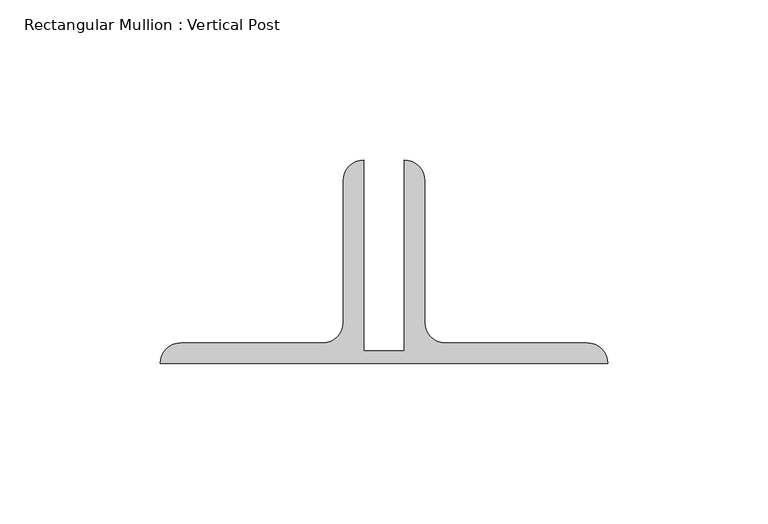
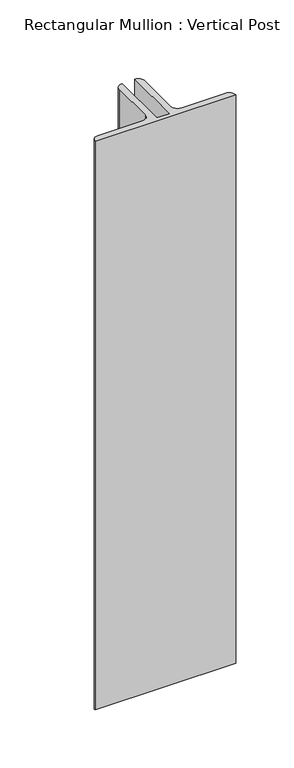
"""IFC4 building model written with IfcOpenShell, lengths in millimetres: member geometry, Rectangular Mullion : Vertical Post."""

from ifc_helpers import new_model, si_unit, point, frame, frame_2d, origin, place, context, project, spatial, polyline, circle_curve, trimmed, segment, composite_curve, outline, extrude, source, transform, mapped, element, save


def rectangular_mullion_vertical_post_a50c0036(model_context):
    return source(origin(), model_context, "Body", "SweptSolid", [
        extrude(outline(composite_curve([segment(polyline([(-6.35, 22.9145205), (6.35, 22.9145205), (6.35, 82.55)]), True, "CONTINUOUS"), segment(trimmed(circle_curve(frame_2d((6.35, 76.2)), 6.35), [point((6.35, 82.55))], [point((12.7, 76.2))], False, "CARTESIAN"), True, "CONTINUOUS"), segment(polyline([(12.7, 76.2), (12.7, 31.75)]), True, "CONTINUOUS"), segment(trimmed(circle_curve(frame_2d((19.05, 31.75)), 6.35), [point((12.7, 31.75))], [point((19.05, 25.4))], True, "CARTESIAN"), True, "CONTINUOUS"), segment(polyline([(19.05, 25.4), (63.5, 25.4)]), True, "CONTINUOUS"), segment(trimmed(circle_curve(frame_2d((63.5, 19.05)), 6.35), [point((63.5, 25.4))], [point((69.85, 19.05))], False, "CARTESIAN"), True, "CONTINUOUS"), segment(polyline([(69.85, 19.05), (-69.85, 19.05)]), True, "CONTINUOUS"), segment(trimmed(circle_curve(frame_2d((-63.5, 19.05)), 6.35), [point((-69.85, 19.05))], [point((-63.5, 25.4))], False, "CARTESIAN"), True, "CONTINUOUS"), segment(polyline([(-63.5, 25.4), (-19.05, 25.4)]), True, "CONTINUOUS"), segment(trimmed(circle_curve(frame_2d((-19.05, 31.75)), 6.35), [point((-19.05, 25.4))], [point((-12.7, 31.75))], True, "CARTESIAN"), True, "CONTINUOUS"), segment(polyline([(-12.7, 31.75), (-12.7, 76.2)]), True, "CONTINUOUS"), segment(trimmed(circle_curve(frame_2d((-6.35, 76.2)), 6.35), [point((-12.7, 76.2))], [point((-6.35, 82.55))], False, "CARTESIAN"), True, "CONTINUOUS"), segment(polyline([(-6.35, 82.55), (-6.35, 22.9145205)]), True, "CONTINUOUS")], self_intersect=False)), frame((0.0, 0.0, -596.9), z_axis=(0.0, 0.0, 1.0), x_axis=(1.0, 0.0, 0.0)), (0.0, 0.0, 1.0), 596.9),
    ])


if __name__ == "__main__":
    model = new_model("IFC4")
    model_context = context("Model", 3, world=origin())
    ifc_project = project(units=[si_unit("LENGTHUNIT", "METRE", prefix="MILLI")], contexts=[model_context])
    site = spatial("IfcSite", under=ifc_project)
    building = spatial("IfcBuilding", under=site)
    placement = place(None, origin())
    rectangular_mullion_vertical_post_shape = rectangular_mullion_vertical_post_a50c0036(model_context)
    element("IfcMember", 1, ObjectType="Rectangular Mullion : Vertical Post", at=placement, inside=building, context=model_context, shape_type="MappedRepresentation", body=[
        mapped(rectangular_mullion_vertical_post_shape, transform((0.0, 0.0, 0.0), x_axis=(1.0, 0.0, 0.0), y_axis=(0.0, 1.0, 0.0), z_axis=(0.0, 0.0, 1.0))),
    ])
    save(model, "model.ifc")

# Revit data of these elements
# Type "Rectangular Mullion : Vertical Post"
#   built-in parameter 1007351 = -0.0625 (stored number, unit not read)
#   built-in parameter 1007322 = 0.0126789 (stored number, unit not read)
#   built-in parameter 1007321 = 0.229167 (stored number, unit not read)
#   built-in parameter 1007320 = 0.229167 (stored number, unit not read)
# Element 1 (IfcMember, "Rectangular Mullion : Vertical Post")
#   Materials on its faces: "GATE POST: (2) BACK/BACK GALVANIZED ANGLES"
# Materials
#   "GATE POST: (2) BACK/BACK GALVANIZED ANGLES": class "Unassigned", colour RGB 211 211 211, transparency 0, Cost = 0
